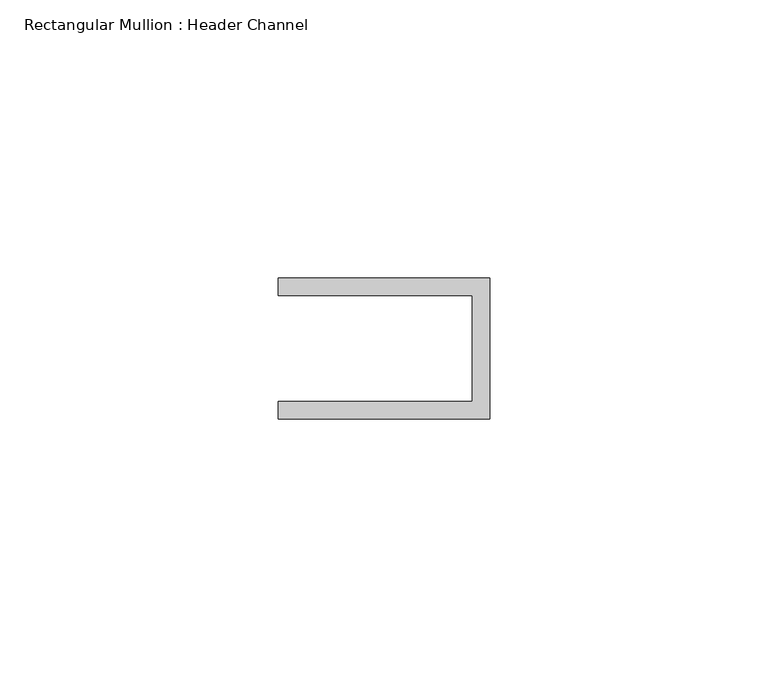
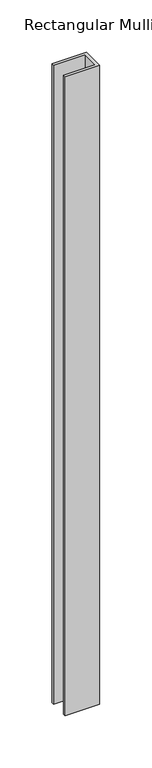
"""IFC4 building model written with IfcOpenShell, lengths in millimetres: member geometry, Rectangular Mullion : Header Channel."""

from ifc_helpers import new_model, si_unit, frame, origin, place, context, project, spatial, polyline, outline, extrude, source, transform, mapped, element, save


def rectangular_mullion_header_channel_7adf1b7f(model_context):
    return source(origin(), model_context, "Body", "SweptSolid", [
        extrude(outline(polyline([(0.0, -12.7), (-38.1, -12.7), (-38.1, -9.525), (-3.175, -9.525), (-3.175, 9.525), (-38.1, 9.525), (-38.1, 12.7), (0.0, 12.7), (0.0, -12.7)])), frame((0.0, 0.0, -747.1996433), z_axis=(0.0, 0.0, 1.0), x_axis=(1.0, 0.0, 0.0)), (0.0, 0.0, 1.0), 747.1996433),
    ])


if __name__ == "__main__":
    model = new_model("IFC4")
    model_context = context("Model", 3, world=origin())
    ifc_project = project(units=[si_unit("LENGTHUNIT", "METRE", prefix="MILLI")], contexts=[model_context])
    site = spatial("IfcSite", under=ifc_project)
    building = spatial("IfcBuilding", under=site)
    placement = place(None, origin())
    rectangular_mullion_header_channel_shape = rectangular_mullion_header_channel_7adf1b7f(model_context)
    element("IfcMember", 1, ObjectType="Rectangular Mullion : Header Channel", at=placement, inside=building, context=model_context, shape_type="MappedRepresentation", body=[
        mapped(rectangular_mullion_header_channel_shape, transform((0.0, 0.0, 0.0), x_axis=(1.0, 0.0, 0.0), y_axis=(0.0, 1.0, 0.0), z_axis=(0.0, 0.0, 1.0))),
    ])
    save(model, "model.ifc")

# Revit data of these elements
# Type "Rectangular Mullion : Header Channel"
#   built-in parameter 1007322 = 0.0833333 (stored number, unit not read)
#   built-in parameter 1007321 = -0.03125 (stored number, unit not read)
#   built-in parameter 1007320 = 0.0416667 (stored number, unit not read)
# Element 1 (IfcMember, "Rectangular Mullion : Header Channel")
#   Materials on its faces: "ALUM"
# Materials
#   "ALUM": class "Generic", colour RGB 157 157 157, transparency 0, Cost = 0
